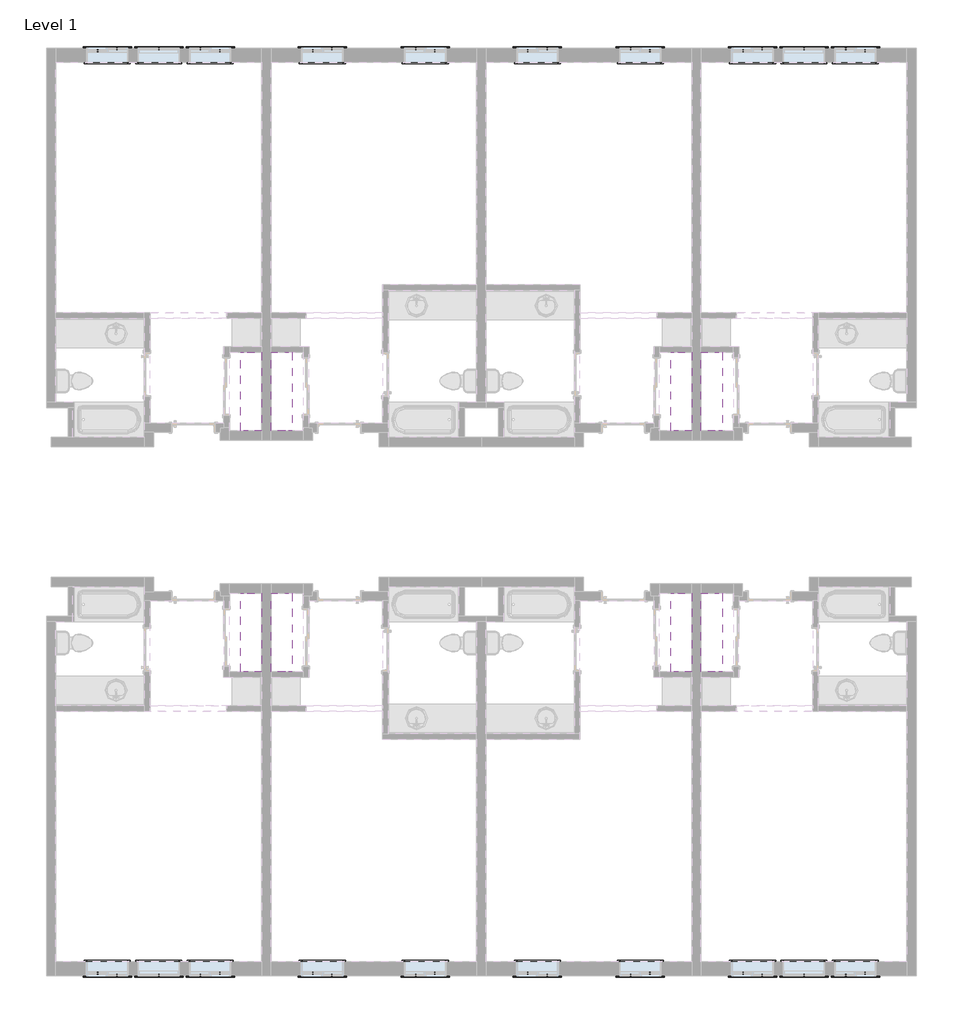
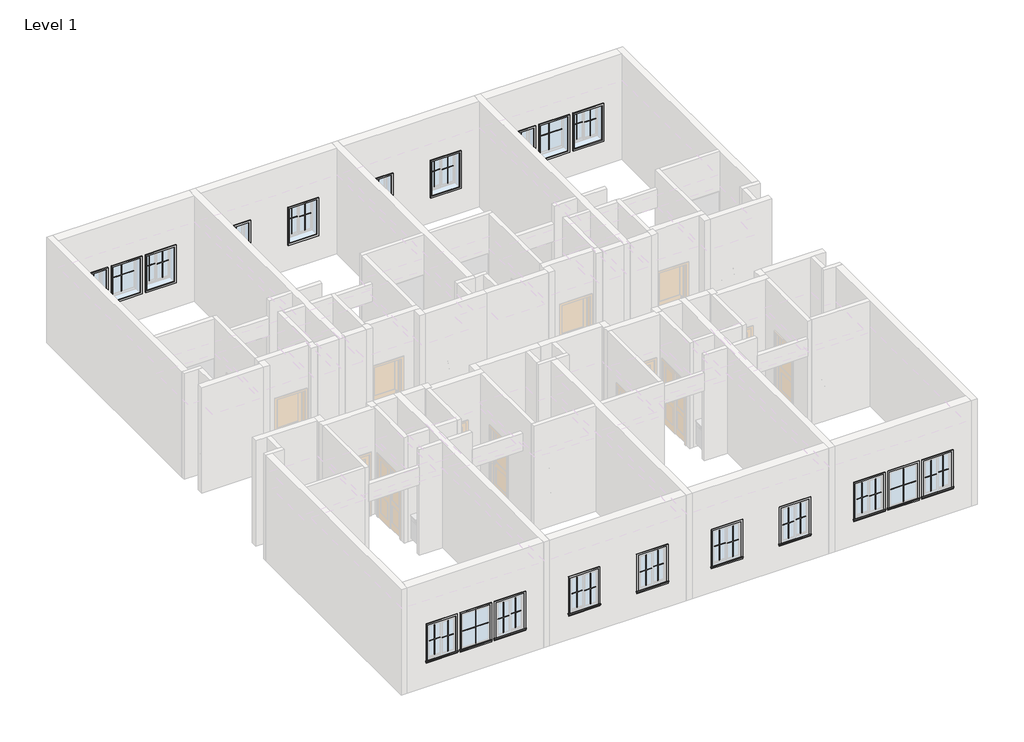
# One storey, part 5 of 5: 84 proxies.
# Revit data of these elements (continued)
# Elements 1, 2, 3, 4, 5, 6, 7, 8 (IfcBuildingElementProxy, "Closet Shelf and Pole : 18\" Deep")
#   built-in parameter 1001306 = 5.58333 (stored number, unit not read)
#   Phase Created = New Construction
#   Materials on its faces: "Birch"
# Elements 9, 10, 43, 44 (IfcBuildingElementProxy, "Muntin Pattern_2x2 : Muntin Pattern_2x2")
#   Width = 2' - 9"
#   Height = 3' - 9"
#   Interior Material = Wood - Stained
#   Exterior Material = Clad - White
#   Phase Created = New Construction
#   Materials on its faces: "Clad - White", "Wood - Stained"
# Elements 11, 12, 13, 14, 15, 16, 17, 18, 19, 20, 21, 22, 23, 24, 25, 26, 27, 28, 29, 30, 31, 32, 33, 34, 35, 36, 37, 38, 39, 40, 41, 42 (IfcBuildingElementProxy, "Muntin Pattern_2x2 : Muntin Pattern_2x2")
#   Width = 1' - 2 5/8"
#   Height = 3' - 6 1/4"
#   Interior Material = Wood - Stained
#   Exterior Material = Clad - White
#   Phase Created = New Construction
#   Materials on its faces: "Clad - White", "Wood - Stained"
# Elements 45, 46, 47, 48, 49, 50, 51, 52, 53, 54, 55, 56, 57, 58, 59, 60, 61, 62, 63, 64 (IfcBuildingElementProxy, "Trim-Window-Exterior-Flat : with Sill")
#   Opening Width = 3' - 0"
#   Opening Height = 4' - 0"
#   Trim Material = Clad - White
#   Phase Created = New Construction
#   Materials on its faces: "Clad - White"
# Elements 65, 66, 67, 68, 69, 70, 71, 72, 73, 74, 75, 76, 77, 78, 79, 80, 81, 82, 83, 84 (IfcBuildingElementProxy, "Trim-Window-Interior-Flat : Picture Frame")
#   Opening Width = 3' - 0"
#   Opening Height = 4' - 0"
#   Trim Material = Wood - Stained
#   Phase Created = New Construction
#   Materials on its faces: "Wood - Stained"
# Materials
#   "Birch": class "Wood", colour RGB 172 132 95, transparency 0, Description = "Betula Alleghaniensis", Cost = 0
#   "Clad - White": class "Wood", colour RGB 242 242 238, transparency 0, Cost = 0
#   "Wood - Stained": class "Wood", colour RGB 224 178 126, transparency 0, Cost = 0
